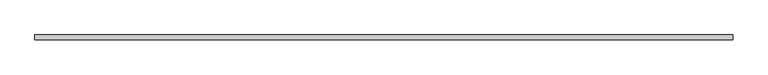
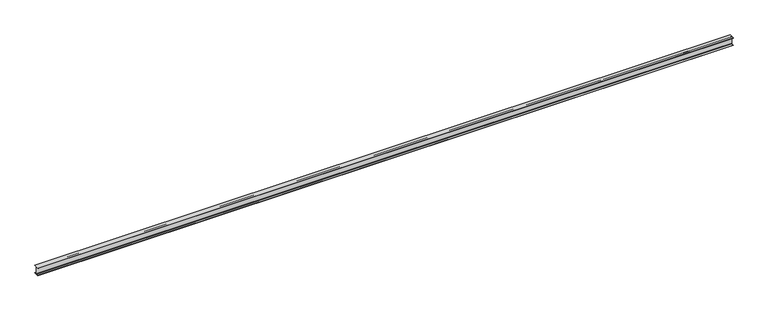
"""IFC4 building model written with IfcOpenShell, lengths in millimetres: beam geometry, Steel Framing_H_KS : H_SB_AR_S02_H-488x300x11x18_CRG1."""

from ifc_helpers import new_model, si_unit, point, frame, frame_2d, origin, place, context, project, spatial, polyline, circle_curve, trimmed, segment, composite_curve, outline, extrude, source, transform, mapped, element, save


def beam_85a0d6c7(model_context):
    return source(origin(), model_context, "Body", "SweptSolid", [
        extrude(outline(composite_curve([segment(polyline([(-150.0, -226.0), (-31.5, -226.0)]), True, "CONTINUOUS"), segment(trimmed(circle_curve(frame_2d((-31.5, -200.0)), 26.0), [point((-31.5, -226.0))], [point((-5.5, -200.0))], True, "CARTESIAN"), True, "CONTINUOUS"), segment(polyline([(-5.5, -200.0), (-5.5, 200.0)]), True, "CONTINUOUS"), segment(trimmed(circle_curve(frame_2d((-31.5, 200.0)), 26.0), [point((-5.5, 200.0))], [point((-31.5, 226.0))], True, "CARTESIAN"), True, "CONTINUOUS"), segment(polyline([(-31.5, 226.0), (-150.0, 226.0), (-150.0, 244.0), (150.0, 244.0), (150.0, 226.0), (31.5, 226.0)]), True, "CONTINUOUS"), segment(trimmed(circle_curve(frame_2d((31.5, 200.0)), 26.0), [point((31.5, 226.0))], [point((5.5, 200.0))], True, "CARTESIAN"), True, "CONTINUOUS"), segment(polyline([(5.5, 200.0), (5.5, -200.0)]), True, "CONTINUOUS"), segment(trimmed(circle_curve(frame_2d((31.5, -200.0)), 26.0), [point((5.5, -200.0))], [point((31.5, -226.0))], True, "CARTESIAN"), True, "CONTINUOUS"), segment(polyline([(31.5, -226.0), (150.0, -226.0), (150.0, -244.0), (-150.0, -244.0), (-150.0, -226.0)]), True, "CONTINUOUS")], self_intersect=False)), frame((-20987.2, 0.0, 0.0), z_axis=(1.0, 0.0, 0.0), x_axis=(0.0, 1.0, 0.0)), (0.0, 0.0, 1.0), 41974.4),
    ])


if __name__ == "__main__":
    model = new_model("IFC4")
    model_context = context("Model", 3, world=origin())
    ifc_project = project(units=[si_unit("LENGTHUNIT", "METRE", prefix="MILLI")], contexts=[model_context])
    site = spatial("IfcSite", under=ifc_project)
    building = spatial("IfcBuilding", under=site)
    placement = place(None, origin())
    beam_shape = beam_85a0d6c7(model_context)
    element("IfcBeam", 1, ObjectType="Steel Framing_H_KS : H_SB_AR_S02_H-488x300x11x18_CRG1", at=placement, inside=building, context=model_context, shape_type="MappedRepresentation", body=[
        mapped(beam_shape, transform((0.0, 0.0, 0.0), x_axis=(1.0, 0.0, 0.0), y_axis=(0.0, 1.0, 0.0), z_axis=(0.0, 0.0, 1.0))),
    ])
    save(model, "model.ifc")

# Revit data of these elements
# Type "Steel Framing_H_KS : H_SB_AR_S02_H-488x300x11x18_CRG1"
#   Type Comments = "MAIN"
#   Type Mark = "CRG1"
#   H_SectionID = "H-488x300x11x18"
#   H_Ratio for Additional Steel Plate = 0.2
#   Width = 30.0 cm
#   Web Thickness = 1.1 cm
#   Web Fillet = 2.6 cm
#   Warping Constant = 4470000.0 cm⁶
#   Torsional Moment of Inertia = 137.492 cm⁴
#   Section Area = 163.5 cm²
#   Plastic Modulus weak axis = 830.0 cm³
#   Plastic Modulus strong axis = 3230.0 cm³
#   Perimeter = 2.11 m²/m
#   Nominal Weight = 128.00 kgf/m
#   Moment of Inertia weak axis = 8110.00 cm⁴
#   Moment of Inertia strong axis = 71000.00 cm⁴
#   Height = 48.8 cm
#   Flange Thickness = 1.8 cm
#   Elastic Modulus weak axis = 541.0 cm³
#   Elastic Modulus strong axis = 2910.0 cm³
#   Centroid Vertical = 24.4 cm
#   Centroid Horizontal = 15.0 cm
#   Bolt Spacing = 8.89 cm
#   Length [instance default] = 1500 mm
#   Structural Material [instance default] = Steel, 45-345
#   Section Name Key = ""
#   Assembly Code = ""
# Element 1 (IfcBeam, "Steel Framing_H_KS : H_SB_AR_S02_H-488x300x11x18_CRG1")
#   Materials on its faces: "Steel, 45-345"
# Materials
#   "Steel, 45-345": class "Metal", colour RGB 189 187 185, transparency 0, Description = "Steel 345 MPa", Cost = 0
